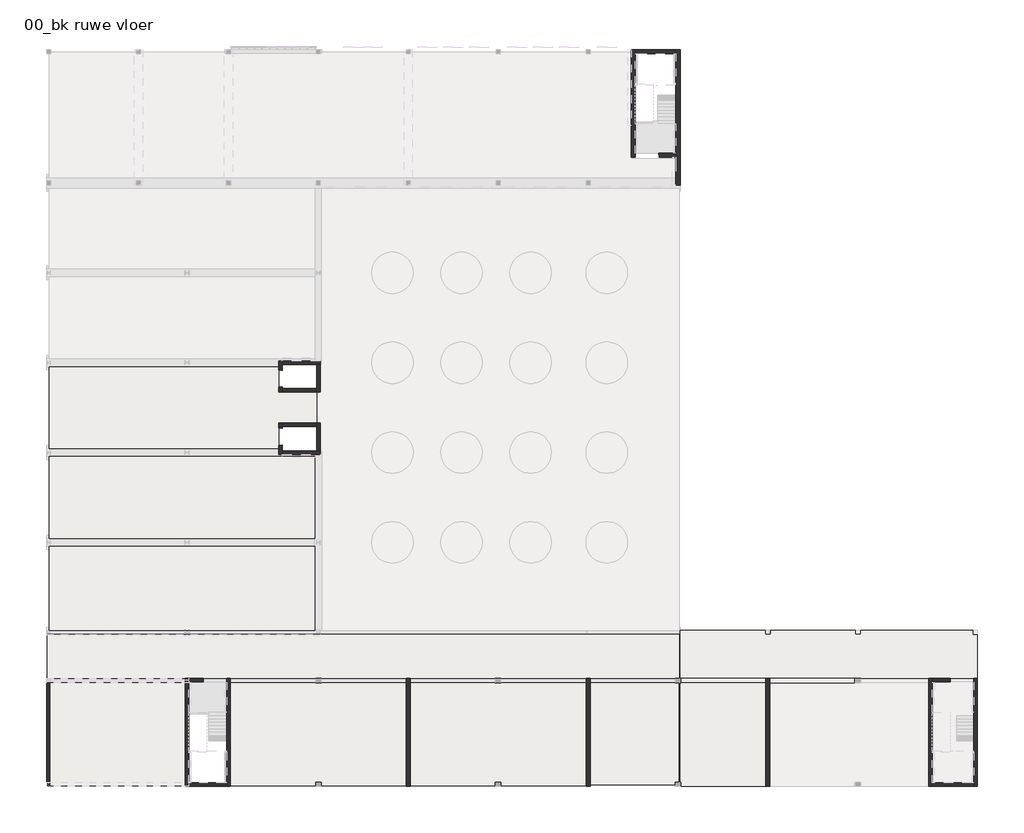
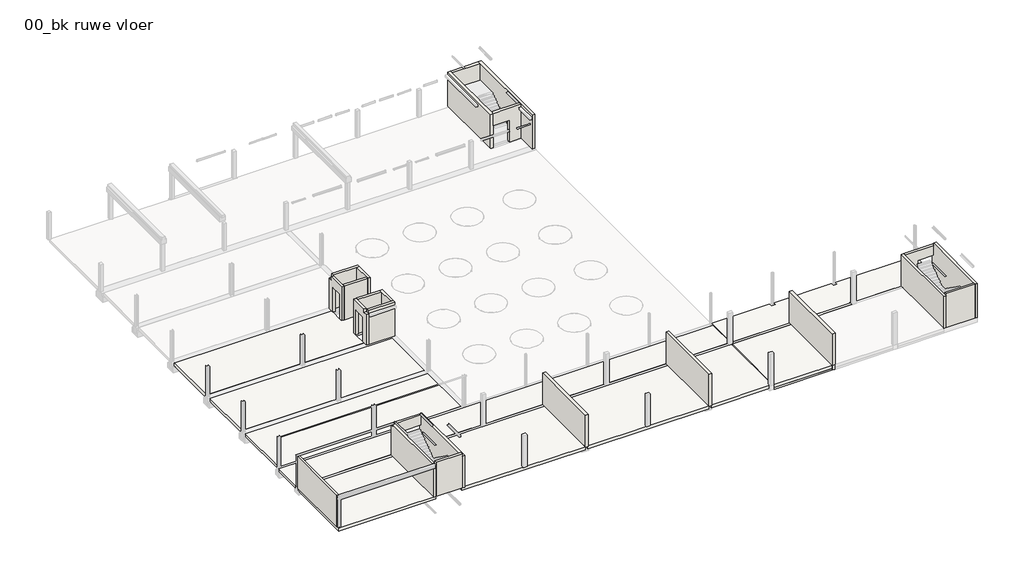
# One storey, part 1 of 6: 24 walls, 18 slabs.
# Revit data of these elements (continued)
# Element 35 (IfcWall, "NLRS_22_WA_beton prefab 250_gen_rsf") (continued)
#   LoadBearing = yes
#   Phase Created = NLRS_nieuw
#   Base Constraint = 00_bk ruwe vloer
#   Top Constraint = 01_bk. ruwe vloer
#   Materials on its faces: "NLRS_f2_beton prefab_gen_rsf"
# Element 36 (IfcWall, "NLRS_22_WA_beton prefab 250_gen_rsf")
#   IfcGUID = "2GRbcre991teoKeCLB8Lp2"
#   built-in parameter 1001111 = 30 mm
#   Top Offset = 0 mm
#   Base Offset = 30 mm
#   wall height = 3770 mm
#   IsExternal = no
#   LoadBearing = yes
#   Phase Created = NLRS_nieuw
#   Base Constraint = 00_bk ruwe vloer
#   Top Constraint = 01_bk. ruwe vloer
#   Materials on its faces: "NLRS_f2_beton prefab_gen_rsf"
# Element 37 (IfcWall, "NLRS_22_WA_beton prefab 250_gen_rsf")
#   IfcGUID = "2GRbcre991teoKeCLB8LoQ"
#   built-in parameter 1001111 = 30 mm
#   Top Offset = 0 mm
#   Base Offset = 30 mm
#   wall height = 3770 mm
#   IsExternal = no
#   LoadBearing = yes
#   Phase Created = NLRS_nieuw
#   Base Constraint = 00_bk ruwe vloer
#   Top Constraint = 01_bk. ruwe vloer
#   Materials on its faces: "NLRS_f2_beton prefab_gen_rsf"
# Element 38 (IfcWall, "NLRS_21_WA_beton prefab 250_gen_rsf")
#   IfcGUID = "2GRbcre991teoKeCLB8LnQ"
#   built-in parameter 1001111 = 30 mm
#   Top Offset = 0 mm
#   Base Offset = 30 mm
#   wall height = 3770 mm
#   IsExternal = yes
#   LoadBearing = yes
#   Phase Created = NLRS_nieuw
#   Base Constraint = 00_bk ruwe vloer
#   Top Constraint = 01_bk. ruwe vloer
#   Materials on its faces: "NLRS_f2_beton prefab_gen_rsf"
# Element 39 (IfcWall, "NLRS_22_WA_beton prefab 250_gen_rsf")
#   IfcGUID = "2GRbcre991teoKeCLB8Lfd"
#   built-in parameter 1001111 = 30 mm
#   Top Offset = 0 mm
#   Base Offset = 30 mm
#   wall height = 3770 mm
#   IsExternal = no
#   LoadBearing = yes
#   Phase Created = NLRS_nieuw
#   Base Constraint = 00_bk ruwe vloer
#   Top Constraint = 01_bk. ruwe vloer
#   Materials on its faces: "NLRS_f2_beton prefab_gen_rsf"
# Element 40 (IfcWall, "NLRS_22_WA_beton prefab 250_gen_rsf")
#   IfcGUID = "2GRbcre991teoKeCLB8Lfb"
#   built-in parameter 1001111 = 30 mm
#   Top Offset = 0 mm
#   Base Offset = 30 mm
#   wall height = 3770 mm
#   IsExternal = no
#   LoadBearing = yes
#   Phase Created = NLRS_nieuw
#   Base Constraint = 00_bk ruwe vloer
#   Top Constraint = 01_bk. ruwe vloer
#   Materials on its faces: "NLRS_f2_beton prefab_gen_rsf"
# Element 41 (IfcWall, "NLRS_22_WA_beton prefab 250_gen_rsf")
#   IfcGUID = "2GRbcre991teoKeCLB8LfZ"
#   built-in parameter 1001111 = 30 mm
#   Top Offset = 0 mm
#   Base Offset = 30 mm
#   wall height = 3770 mm
#   IsExternal = no
#   LoadBearing = yes
#   Phase Created = NLRS_nieuw
#   Base Constraint = 00_bk ruwe vloer
#   Top Constraint = 01_bk. ruwe vloer
#   Materials on its faces: "NLRS_f2_beton prefab_gen_rsf"
# Element 42 (IfcWall, "NLRS_21_WA_beton prefab 250_gen_rsf")
#   IfcGUID = "2GRbcre991teoKeCLB8LfX"
#   built-in parameter 1001111 = 30 mm
#   Top Offset = 0 mm
#   Base Offset = 30 mm
#   wall height = 3770 mm
#   IsExternal = yes
#   LoadBearing = yes
#   Phase Created = NLRS_nieuw
#   Base Constraint = 00_bk ruwe vloer
#   Top Constraint = 01_bk. ruwe vloer
#   Materials on its faces: "NLRS_f2_beton prefab_gen_rsf"
# Materials
#   "NLRS_f2_beton prefab_gen_rsf": class "F - Niet gebakken kunststeen", colour RGB 129 133 118, transparency 0, Keynote = "f2", Manufacturer = "Revit Standards Foundation", URL = "www.revitstandards.org", Description = "beton prefab", Cost = 0
#   "NLRS_f2_beton ihwg_gen_rsf": class "F - Niet gebakken kunststeen", colour RGB 129 133 118, transparency 0, Keynote = "f2", Manufacturer = "Revit Standards Foundation", URL = "www.revitstandards.org", Description = "beton ihwg", Cost = 0
#   "NLRS_n7_isolatie EPS_gen_rsf": class "N - Kunststoffen, rubbers", colour RGB 200 200 140, transparency 0, Keynote = "n7", Manufacturer = "Revit Standards Foundation", URL = "www.revitstandards.org", Description = "isolatie EPS", Cost = 0
#   "NLRS_f1_kalkzandsteen_gen_rsf": class "F - Niet gebakken kunststeen", colour RGB 223 221 219, transparency 0, Keynote = "f1", Manufacturer = "Revit Standards Foundation", URL = "www.revitstandards.org", Description = "kalkzandsteen", Cost = 0
# Room, not placed, phase "NLRS_bestaand", upper offset 0 mm, lower offset 0 mm
#   Number = "1"
#   Name = "Room"
